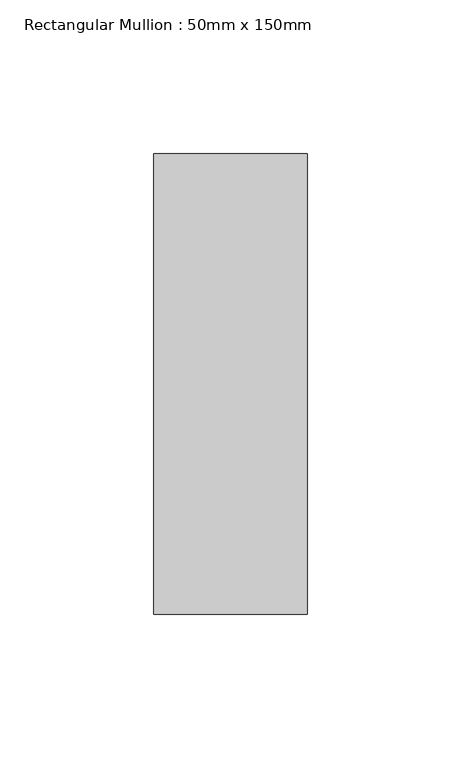
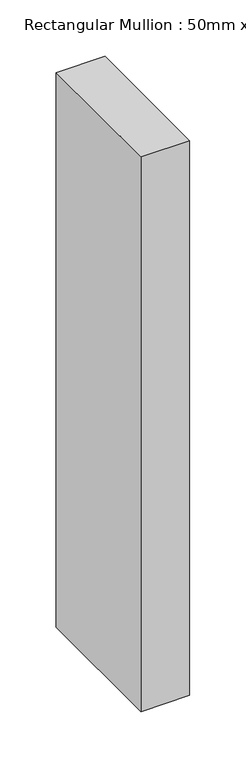
"""IFC4 building model written with IfcOpenShell, lengths in millimetres: member geometry, Rectangular Mullion : 50mm x 150mm."""

from ifc_helpers import new_model, si_unit, frame, origin, place, context, project, spatial, polyline, outline, extrude, source, transform, mapped, element, save


def rectangular_mullion_50mm_x_150mm_64d38db8(model_context):
    return source(origin(), model_context, "Body", "SweptSolid", [
        extrude(outline(polyline([(0.0, 75.0), (0.0, -75.0), (-50.0, -75.0), (-50.0, 75.0), (0.0, 75.0)])), frame((0.0, 0.0, -600.0), z_axis=(0.0, 0.0, 1.0), x_axis=(1.0, 0.0, 0.0)), (0.0, 0.0, 1.0), 600.0),
    ])


if __name__ == "__main__":
    model = new_model("IFC4")
    model_context = context("Model", 3, world=origin())
    ifc_project = project(units=[si_unit("LENGTHUNIT", "METRE", prefix="MILLI")], contexts=[model_context])
    site = spatial("IfcSite", under=ifc_project)
    building = spatial("IfcBuilding", under=site)
    placement = place(None, origin())
    rectangular_mullion_50mm_x_150mm_shape = rectangular_mullion_50mm_x_150mm_64d38db8(model_context)
    element("IfcMember", 1, ObjectType="Rectangular Mullion : 50mm x 150mm", at=placement, inside=building, context=model_context, shape_type="MappedRepresentation", body=[
        mapped(rectangular_mullion_50mm_x_150mm_shape, transform((0.0, 0.0, 0.0), x_axis=(1.0, 0.0, 0.0), y_axis=(0.0, 1.0, 0.0), z_axis=(0.0, 0.0, 1.0))),
    ])
    save(model, "model.ifc")

# Revit data of these elements
# Type "Rectangular Mullion : 50mm x 150mm"
#   built-in parameter 1007304 = 0.492126 (stored number, unit not read)
#   built-in parameter 1007301 = 0.082021 (stored number, unit not read)
#   built-in parameter 1007300 = 0.082021 (stored number, unit not read)
# Element 1 (IfcMember, "Rectangular Mullion : 50mm x 150mm")
#   Materials on its faces: "Aluminum"
# Materials
#   "Aluminum": class "Metal", colour RGB 244 244 244, transparency 0, Description = "Aluminum 6061", Cost = 0
